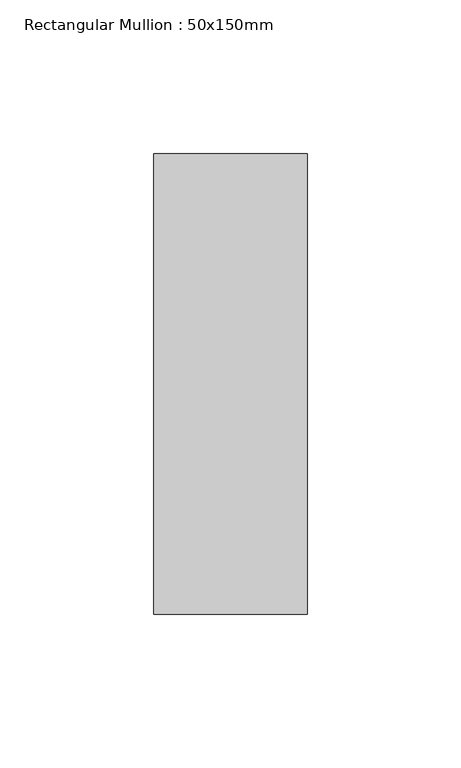
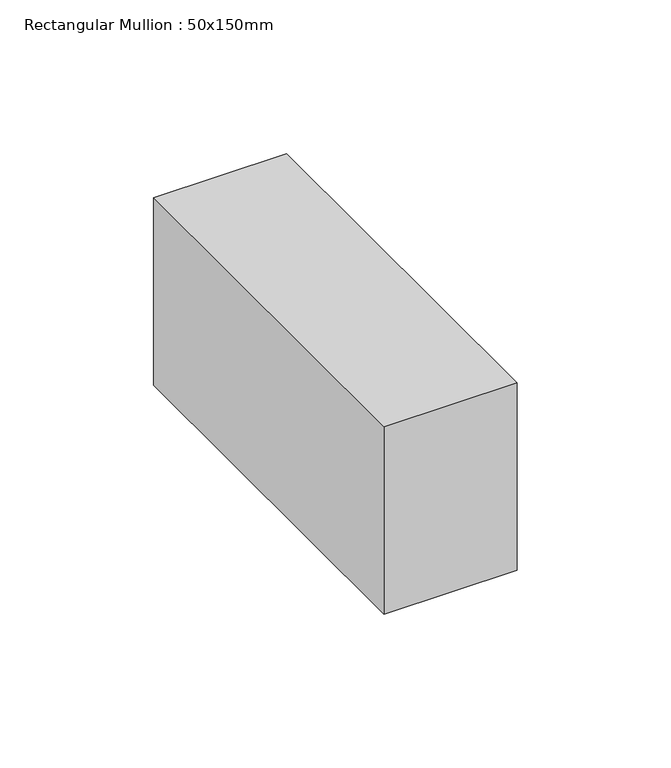
"""IFC4 building model written with IfcOpenShell, lengths in millimetres: member geometry, Rectangular Mullion : 50x150mm."""

import ifcopenshell
import ifcopenshell.guid

model = None  # the IFC model being written
_history = None  # IfcOwnerHistory: only IFC2X3 demands one
_inside = {}  # id of a spatial element -> (the spatial element, [elements in it])
_under = {}  # id of a project, library or spatial element -> (it, [spatial elements below it])
_declared = {}  # id of a project -> (the project, [libraries it declares])
_typed = {}  # id of a type object -> (the type object, [elements of that type])
_made_of = {}  # id of a material, layer set ... -> (it, [elements and type objects made of it])


def new_model(schema):
    """Start an empty IFC model of exactly this schema.

    Asked for "IFC4X3", IfcOpenShell would pick the latest addendum, in which some entities
    have other attributes; the version numbers below select the first issue.
    IFC2X3 requires an IfcOwnerHistory on every rooted entity: one is made here for all.
    """
    global model, _history
    if schema == "IFC4X3":
        model = ifcopenshell.file(schema_version=(4, 3, 0, 0))
    else:
        model = ifcopenshell.file(schema=schema)
    _inside.clear()
    _under.clear()
    _declared.clear()
    _typed.clear()
    _made_of.clear()
    _history = None
    if model.schema == "IFC2X3":
        org = make("IfcOrganization", Name="unknown")
        user = make(
            "IfcPersonAndOrganization",
            ThePerson=make("IfcPerson", FamilyName="unknown"),
            TheOrganization=org,
        )
        app = make(
            "IfcApplication",
            ApplicationDeveloper=org,
            Version="unknown",
            ApplicationFullName="unknown",
            ApplicationIdentifier="unknown",
        )
        _history = make(
            "IfcOwnerHistory",
            OwningUser=user,
            OwningApplication=app,
            ChangeAction="ADDED",
            CreationDate=0,
        )
    return model


def make(cls, **values):
    """One entity of the class cls with the attributes given. An attribute that is None is left unset."""
    return model.create_entity(
        cls, **{name: value for name, value in values.items() if value is not None}
    )


def rooted(cls, **values):
    """An entity with a GlobalId (a new one), such as an element, a storey or a relation."""
    return make(cls, GlobalId=ifcopenshell.guid.new(), OwnerHistory=_history, **values)


def si_unit(unit_type, name, prefix=None):
    """IfcSIUnit, for example si_unit("LENGTHUNIT", "METRE", prefix="MILLI")."""
    return make("IfcSIUnit", UnitType=unit_type, Prefix=prefix, Name=name)


def assignment(units):
    """IfcUnitAssignment: the units of a project."""
    return None if units is None else make("IfcUnitAssignment", Units=units)


def point(xyz):
    """IfcCartesianPoint."""
    return None if xyz is None else make("IfcCartesianPoint", Coordinates=xyz)


def direction(xyz):
    """IfcDirection."""
    return None if xyz is None else make("IfcDirection", DirectionRatios=xyz)


def frame(location, z_axis=None, x_axis=None):
    """IfcAxis2Placement3D, a coordinate frame: its origin and axes. An axis left out is left unset."""
    return make(
        "IfcAxis2Placement3D",
        Location=point(location),
        Axis=direction(z_axis),
        RefDirection=direction(x_axis),
    )


def origin():
    """The frame at (0, 0, 0) with its axes left unset."""
    return frame((0.0, 0.0, 0.0))


def place(relative_to, where):
    """IfcLocalPlacement: puts the frame where relative to a parent placement (None: the world)."""
    return make(
        "IfcLocalPlacement", PlacementRelTo=relative_to, RelativePlacement=where
    )


def context(
    kind, dimensions, precision=None, world=None, true_north=None, identifier=None
):
    """IfcGeometricRepresentationContext, for example the 3D "Model" context."""
    return make(
        "IfcGeometricRepresentationContext",
        ContextIdentifier=identifier,
        ContextType=kind,
        CoordinateSpaceDimension=dimensions,
        Precision=precision,
        WorldCoordinateSystem=world,
        TrueNorth=true_north,
    )


def project(units=None, contexts=None):
    """IfcProject with its units and contexts."""
    return rooted(
        "IfcProject",
        Name="project",
        RepresentationContexts=contexts,
        UnitsInContext=assignment(units),
    )


def spatial(cls, under=None, at=None, **own):
    """A site, building, storey or space (cls), placed at a placement, below another one or the project."""
    s = rooted(cls, ObjectPlacement=at, **own)
    if under is not None:
        _under.setdefault(under.id(), (under, []))[1].append(s)
    return s


def polyline(points):
    """IfcPolyline through the points."""
    return make("IfcPolyline", Points=[point(p) for p in points])


def outline(outer, holes=None, kind="AREA"):
    """IfcArbitraryClosedProfileDef: a profile drawn as a closed curve; with holes, ...WithVoids."""
    if holes is None:
        return make("IfcArbitraryClosedProfileDef", ProfileType=kind, OuterCurve=outer)
    return make(
        "IfcArbitraryProfileDefWithVoids",
        ProfileType=kind,
        OuterCurve=outer,
        InnerCurves=holes,
    )


def extrude(swept, where, along, depth):
    """IfcExtrudedAreaSolid: the profile swept, set in the frame where, extruded along a direction by depth."""
    return make(
        "IfcExtrudedAreaSolid",
        SweptArea=swept,
        Position=where,
        ExtrudedDirection=direction(along),
        Depth=depth,
    )


def shape(context_of_items, identifier, shape_type, items):
    """IfcShapeRepresentation: the items that make up one representation, for example the "Body"."""
    return make(
        "IfcShapeRepresentation",
        ContextOfItems=context_of_items,
        RepresentationIdentifier=identifier,
        RepresentationType=shape_type,
        Items=items,
    )


def source(mapping_origin, context_of_items, identifier, shape_type, items):
    """IfcRepresentationMap: a shape defined once, which mapped items show again and again."""
    return make(
        "IfcRepresentationMap",
        MappingOrigin=mapping_origin,
        MappedRepresentation=shape(context_of_items, identifier, shape_type, items),
    )


def transform(
    local_origin,
    x_axis=None,
    y_axis=None,
    z_axis=None,
    scale=None,
    scale2=None,
    scale3=None,
    uniform=True,
):
    """IfcCartesianTransformationOperator3D, or its non-uniform kind. x_axis, y_axis, z_axis: its Axis1, 2, 3."""
    if uniform:
        return make(
            "IfcCartesianTransformationOperator3D",
            Axis1=direction(x_axis),
            Axis2=direction(y_axis),
            LocalOrigin=point(local_origin),
            Scale=scale,
            Axis3=direction(z_axis),
        )
    return make(
        "IfcCartesianTransformationOperator3DnonUniform",
        Axis1=direction(x_axis),
        Axis2=direction(y_axis),
        LocalOrigin=point(local_origin),
        Scale=scale,
        Axis3=direction(z_axis),
        Scale2=scale2,
        Scale3=scale3,
    )


def mapped(mapping_source, mapping_target):
    """IfcMappedItem: shows the shape of a source again, moved by a transform."""
    return make(
        "IfcMappedItem", MappingSource=mapping_source, MappingTarget=mapping_target
    )


def made_of(thing, what):
    """Note that an element or type object is made of a material, layer set ...; save() writes the relation."""
    if what is not None:
        _made_of.setdefault(what.id(), (what, []))[1].append(thing)
    return thing


def element(
    cls,
    number,
    at=None,
    inside=None,
    cuts=None,
    type_object=None,
    material=None,
    context=None,
    identifier="Body",
    shape_type=None,
    held_by="IfcProductDefinitionShape",
    body=None,
    shapes=None,
    **own,
):
    """One element of the class cls, such as IfcWall. Its Tag is "e" and its number.

    at: its placement. inside: the storey or other place that contains it. cuts: it is an
    opening in that element (IfcRelVoidsElement). A single representation is given by context,
    identifier, shape_type and body (its items); several are given by shapes. held_by: the class
    of the entity that holds the representations. save() writes the other relations.
    """
    e = rooted(cls, Tag="e%d" % number, ObjectPlacement=at, **own)
    if body is not None:
        shapes = [shape(context, identifier, shape_type, body)]
    if shapes is not None:
        e.Representation = make(held_by, Representations=shapes)
    if inside is not None:
        _inside.setdefault(inside.id(), (inside, []))[1].append(e)
    if cuts is not None:
        rooted(
            "IfcRelVoidsElement", RelatingBuildingElement=cuts, RelatedOpeningElement=e
        )
    if type_object is not None:
        _typed.setdefault(type_object.id(), (type_object, []))[1].append(e)
    return made_of(e, material)


def aggregate(whole, parts):
    """IfcRelAggregates: a whole, such as a stair, and the parts it consists of."""
    return rooted("IfcRelAggregates", RelatingObject=whole, RelatedObjects=parts)


def save(model, path):
    """Write the relations noted so far, then the file.

    IfcRelAggregates (storeys below a building ...), IfcRelContainedInSpatialStructure (elements
    in a storey), IfcRelDefinesByType, IfcRelAssociatesMaterial and IfcRelDeclares: one each for
    every whole, place, type object, material and project.
    """
    for whole, parts in _under.values():
        aggregate(whole, parts)
    for where, things in _inside.values():
        rooted(
            "IfcRelContainedInSpatialStructure",
            RelatedElements=things,
            RelatingStructure=where,
        )
    for kind, things in _typed.values():
        rooted("IfcRelDefinesByType", RelatedObjects=things, RelatingType=kind)
    for what, things in _made_of.values():
        rooted("IfcRelAssociatesMaterial", RelatedObjects=things, RelatingMaterial=what)
    for by, libraries in _declared.values():
        rooted("IfcRelDeclares", RelatingContext=by, RelatedDefinitions=libraries)
    model.write(path)


def rectangular_mullion_50x150mm_6eefbde0(model_context):
    return source(origin(), model_context, "Body", "SweptSolid", [
        extrude(outline(polyline([(0.0, 75.0), (0.0, -75.0), (-50.0, -75.0), (-50.0, 75.0), (0.0, 75.0)])), frame((0.0, 0.0, -74.4185145), z_axis=(0.0, 0.0, 1.0), x_axis=(1.0, 0.0, 0.0)), (0.0, 0.0, 1.0), 74.4185145),
    ])


if __name__ == "__main__":
    model = new_model("IFC4")
    model_context = context("Model", 3, world=origin())
    ifc_project = project(units=[si_unit("LENGTHUNIT", "METRE", prefix="MILLI")], contexts=[model_context])
    site = spatial("IfcSite", under=ifc_project)
    building = spatial("IfcBuilding", under=site)
    placement = place(None, origin())
    rectangular_mullion_50x150mm_shape = rectangular_mullion_50x150mm_6eefbde0(model_context)
    element("IfcMember", 1, ObjectType="Rectangular Mullion : 50x150mm", at=placement, inside=building, context=model_context, shape_type="MappedRepresentation", body=[
        mapped(rectangular_mullion_50x150mm_shape, transform((0.0, 0.0, 0.0), x_axis=(1.0, 0.0, 0.0), y_axis=(0.0, 1.0, 0.0), z_axis=(0.0, 0.0, 1.0))),
    ])
    save(model, "model.ifc")

# Revit data of these elements
# Type "Rectangular Mullion : 50x150mm"
#   Keynote = "H11"
#   built-in parameter 1007304 = 0.492126 (stored number, unit not read)
#   built-in parameter 1007301 = 0.082021 (stored number, unit not read)
#   built-in parameter 1007300 = 0.082021 (stored number, unit not read)
# Element 1 (IfcMember, "Rectangular Mullion : 50x150mm")
#   Materials on its faces: "Aluminium"
# Materials
#   "Aluminium": class "Metal", colour RGB 247 247 247, transparency 0, Description = "Aluminium 6061", Cost = 0
